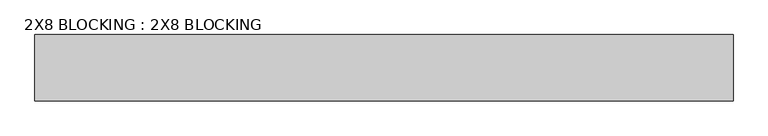
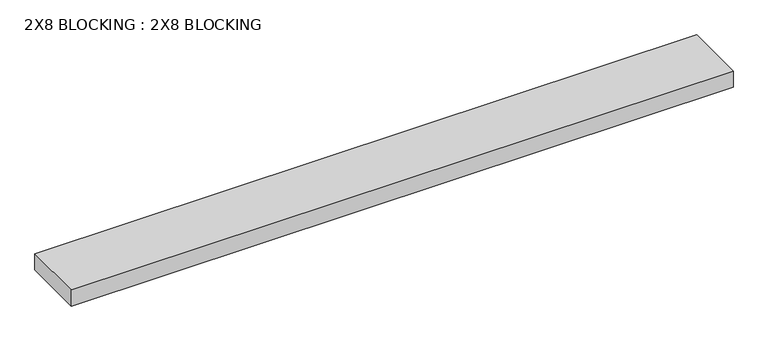
"""IFC4 building model written with IfcOpenShell, lengths in millimetres: proxy geometry, 2X8 BLOCKING : 2X8 BLOCKING."""

from ifc_helpers import new_model, si_unit, frame, origin, place, context, project, spatial, polyline, outline, extrude, source, transform, mapped, element, save


def proxy_2x8_blocking_2x8_blocking_a2a7dfde(model_context):
    return source(origin(), model_context, "Body", "SweptSolid", [
        extrude(outline(polyline([(12382.7678845, -5536.0675368), (12382.7678845, -5345.4245733), (14383.0178845, -5345.4245733), (14383.0178845, -5536.0675368), (12382.7678845, -5536.0675368)])), frame((0.0, 0.0, 40169.0223301), z_axis=(0.0, 0.0, 1.0), x_axis=(1.0, 0.0, 0.0)), (0.0, 0.0, 1.0), 51.9935355),
    ])


if __name__ == "__main__":
    model = new_model("IFC4")
    model_context = context("Model", 3, world=origin())
    ifc_project = project(units=[si_unit("LENGTHUNIT", "METRE", prefix="MILLI")], contexts=[model_context])
    site = spatial("IfcSite", under=ifc_project)
    building = spatial("IfcBuilding", under=site)
    placement = place(None, origin())
    proxy_2x8_blocking_2x8_blocking_shape = proxy_2x8_blocking_2x8_blocking_a2a7dfde(model_context)
    element("IfcBuildingElementProxy", 1, Name="2X8 BLOCKING : 2X8 BLOCKING", ObjectType="2X8 BLOCKING : 2X8 BLOCKING", at=placement, inside=building, context=model_context, shape_type="MappedRepresentation", body=[
        mapped(proxy_2x8_blocking_2x8_blocking_shape, transform((0.0, 0.0, 0.0), x_axis=(1.0, 0.0, 0.0), y_axis=(0.0, 1.0, 0.0), z_axis=(0.0, 0.0, 1.0))),
    ])
    save(model, "model.ifc")

# Revit data of these elements
# Type "2X8 BLOCKING : 2X8 BLOCKING"
#   NameOverride = "2X8 BLOCKING"
# Element 1 (IfcBuildingElementProxy, "2X8 BLOCKING : 2X8 BLOCKING")
#   Materials on its faces: "WOOD BLOCKING AS REQUIRED"
# Materials
#   "WOOD BLOCKING AS REQUIRED": class "Unassigned", colour RGB 166 124 85, transparency 0, Cost = 0
